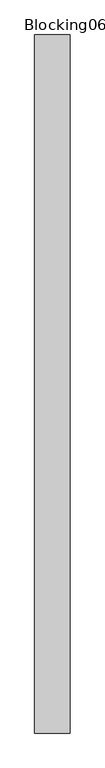
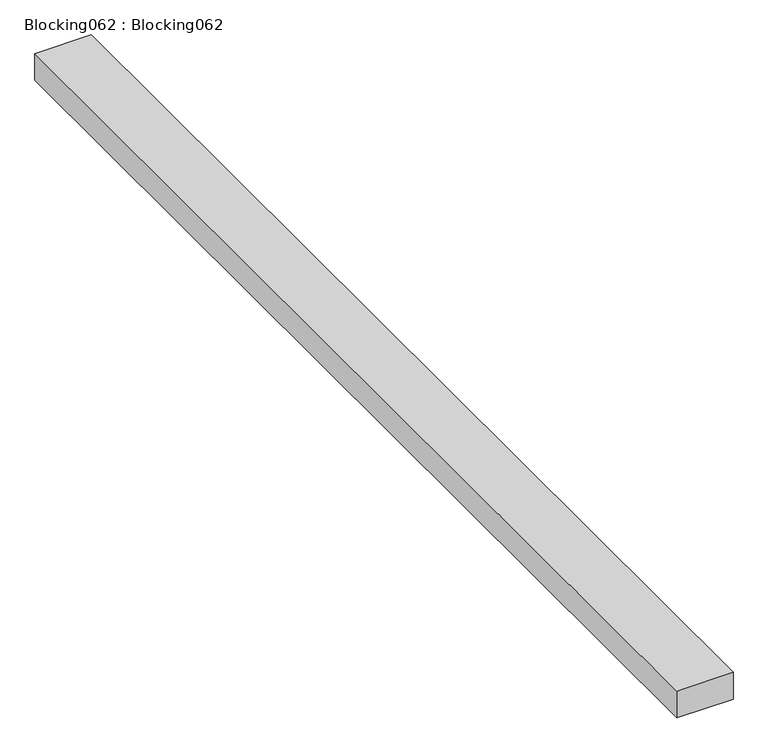
"""IFC4 building model written with IfcOpenShell, lengths in millimetres: proxy geometry, Blocking062 : Blocking062."""

from ifc_helpers import new_model, si_unit, frame, origin, place, context, project, spatial, polyline, outline, extrude, source, transform, mapped, element, save


def blocking062_blocking062_57565c02(model_context):
    return source(origin(), model_context, "Body", "SweptSolid", [
        extrude(outline(polyline([(-7121.5276325, 7982.1531721), (-7223.1276325, 7982.1531721), (-7223.1276325, 9982.1531721), (-7121.5276325, 9982.1531721), (-7121.5276325, 7982.1531721)])), frame((0.0, 0.0, 39953.9460083), z_axis=(0.0, 0.0, 1.0), x_axis=(1.0, 0.0, 0.0)), (0.0, 0.0, 1.0), 50.8),
    ])


if __name__ == "__main__":
    model = new_model("IFC4")
    model_context = context("Model", 3, world=origin())
    ifc_project = project(units=[si_unit("LENGTHUNIT", "METRE", prefix="MILLI")], contexts=[model_context])
    site = spatial("IfcSite", under=ifc_project)
    building = spatial("IfcBuilding", under=site)
    placement = place(None, origin())
    blocking062_blocking062_shape = blocking062_blocking062_57565c02(model_context)
    element("IfcBuildingElementProxy", 1, Name="Blocking062 : Blocking062", ObjectType="Blocking062 : Blocking062", at=placement, inside=building, context=model_context, shape_type="MappedRepresentation", body=[
        mapped(blocking062_blocking062_shape, transform((0.0, 0.0, 0.0), x_axis=(1.0, 0.0, 0.0), y_axis=(0.0, 1.0, 0.0), z_axis=(0.0, 0.0, 1.0))),
    ])
    save(model, "model.ifc")

# Revit data of these elements
# Type "Blocking062 : Blocking062"
#   NameOverride = "Blocking062"
# Element 1 (IfcBuildingElementProxy, "Blocking062 : Blocking062")
#   Materials on its faces: "WOOD BLOCKING AS REQUIRED"
# Materials
#   "WOOD BLOCKING AS REQUIRED": class "Unassigned", colour RGB 166 124 85, transparency 0, Cost = 0
